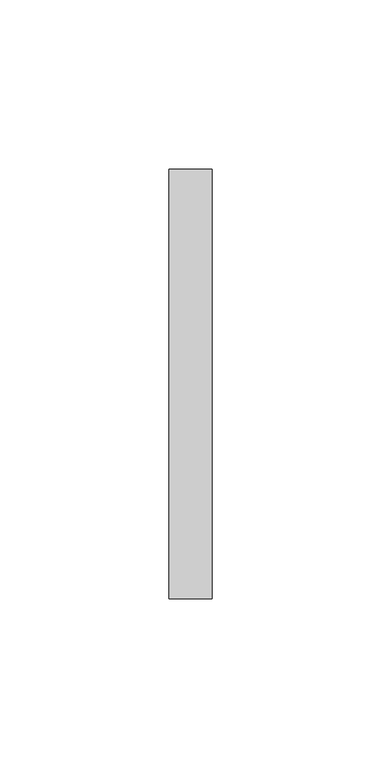
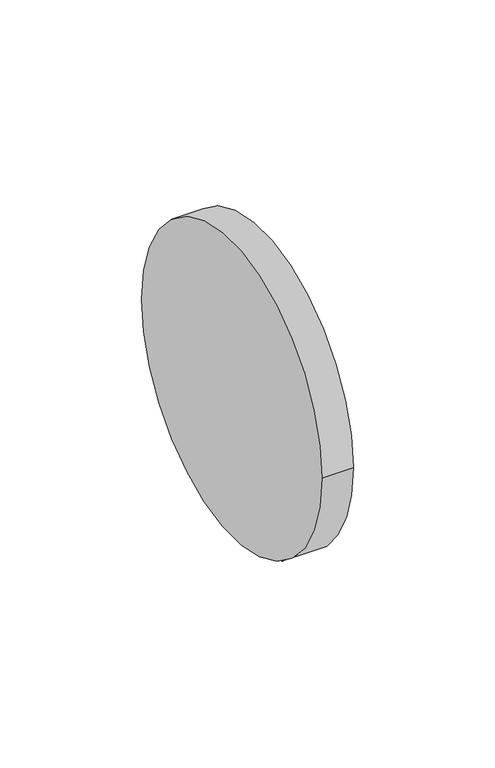
"""IFC4 building model written with IfcOpenShell, lengths in millimetres: proxy geometry, DOAS Supply to Return Connection : DOAS Supply to Return Duct Connection."""

import ifcopenshell
import ifcopenshell.guid

model = None  # the IFC model being written
_history = None  # IfcOwnerHistory: only IFC2X3 demands one
_inside = {}  # id of a spatial element -> (the spatial element, [elements in it])
_under = {}  # id of a project, library or spatial element -> (it, [spatial elements below it])
_declared = {}  # id of a project -> (the project, [libraries it declares])
_typed = {}  # id of a type object -> (the type object, [elements of that type])
_made_of = {}  # id of a material, layer set ... -> (it, [elements and type objects made of it])


def new_model(schema):
    """Start an empty IFC model of exactly this schema.

    Asked for "IFC4X3", IfcOpenShell would pick the latest addendum, in which some entities
    have other attributes; the version numbers below select the first issue.
    IFC2X3 requires an IfcOwnerHistory on every rooted entity: one is made here for all.
    """
    global model, _history
    if schema == "IFC4X3":
        model = ifcopenshell.file(schema_version=(4, 3, 0, 0))
    else:
        model = ifcopenshell.file(schema=schema)
    _inside.clear()
    _under.clear()
    _declared.clear()
    _typed.clear()
    _made_of.clear()
    _history = None
    if model.schema == "IFC2X3":
        org = make("IfcOrganization", Name="unknown")
        user = make(
            "IfcPersonAndOrganization",
            ThePerson=make("IfcPerson", FamilyName="unknown"),
            TheOrganization=org,
        )
        app = make(
            "IfcApplication",
            ApplicationDeveloper=org,
            Version="unknown",
            ApplicationFullName="unknown",
            ApplicationIdentifier="unknown",
        )
        _history = make(
            "IfcOwnerHistory",
            OwningUser=user,
            OwningApplication=app,
            ChangeAction="ADDED",
            CreationDate=0,
        )
    return model


def make(cls, **values):
    """One entity of the class cls with the attributes given. An attribute that is None is left unset."""
    return model.create_entity(
        cls, **{name: value for name, value in values.items() if value is not None}
    )


def rooted(cls, **values):
    """An entity with a GlobalId (a new one), such as an element, a storey or a relation."""
    return make(cls, GlobalId=ifcopenshell.guid.new(), OwnerHistory=_history, **values)


def si_unit(unit_type, name, prefix=None):
    """IfcSIUnit, for example si_unit("LENGTHUNIT", "METRE", prefix="MILLI")."""
    return make("IfcSIUnit", UnitType=unit_type, Prefix=prefix, Name=name)


def assignment(units):
    """IfcUnitAssignment: the units of a project."""
    return None if units is None else make("IfcUnitAssignment", Units=units)


def point(xyz):
    """IfcCartesianPoint."""
    return None if xyz is None else make("IfcCartesianPoint", Coordinates=xyz)


def direction(xyz):
    """IfcDirection."""
    return None if xyz is None else make("IfcDirection", DirectionRatios=xyz)


def frame(location, z_axis=None, x_axis=None):
    """IfcAxis2Placement3D, a coordinate frame: its origin and axes. An axis left out is left unset."""
    return make(
        "IfcAxis2Placement3D",
        Location=point(location),
        Axis=direction(z_axis),
        RefDirection=direction(x_axis),
    )


def frame_2d(location, x_axis=None):
    """IfcAxis2Placement2D, a coordinate frame in the plane: its origin and x axis."""
    return make(
        "IfcAxis2Placement2D", Location=point(location), RefDirection=direction(x_axis)
    )


def origin():
    """The frame at (0, 0, 0) with its axes left unset."""
    return frame((0.0, 0.0, 0.0))


def origin_2d():
    """The frame at (0, 0) in the plane with its x axis left unset."""
    return frame_2d((0.0, 0.0))


def place(relative_to, where):
    """IfcLocalPlacement: puts the frame where relative to a parent placement (None: the world)."""
    return make(
        "IfcLocalPlacement", PlacementRelTo=relative_to, RelativePlacement=where
    )


def context(
    kind, dimensions, precision=None, world=None, true_north=None, identifier=None
):
    """IfcGeometricRepresentationContext, for example the 3D "Model" context."""
    return make(
        "IfcGeometricRepresentationContext",
        ContextIdentifier=identifier,
        ContextType=kind,
        CoordinateSpaceDimension=dimensions,
        Precision=precision,
        WorldCoordinateSystem=world,
        TrueNorth=true_north,
    )


def project(units=None, contexts=None):
    """IfcProject with its units and contexts."""
    return rooted(
        "IfcProject",
        Name="project",
        RepresentationContexts=contexts,
        UnitsInContext=assignment(units),
    )


def spatial(cls, under=None, at=None, **own):
    """A site, building, storey or space (cls), placed at a placement, below another one or the project."""
    s = rooted(cls, ObjectPlacement=at, **own)
    if under is not None:
        _under.setdefault(under.id(), (under, []))[1].append(s)
    return s


def circle_curve(where, radius):
    """IfcCircle in the frame where."""
    return make("IfcCircle", Position=where, Radius=radius)


def trimmed(basis, trim1, trim2, sense, master):
    """IfcTrimmedCurve: the piece of a basis curve between two trims."""
    return make(
        "IfcTrimmedCurve",
        BasisCurve=basis,
        Trim1=trim1,
        Trim2=trim2,
        SenseAgreement=sense,
        MasterRepresentation=master,
    )


def segment(curve, same_sense, transition):
    """IfcCompositeCurveSegment."""
    return make(
        "IfcCompositeCurveSegment",
        Transition=transition,
        SameSense=same_sense,
        ParentCurve=curve,
    )


def composite_curve(segments, self_intersect=None):
    """IfcCompositeCurve: segments joined end to end."""
    return make("IfcCompositeCurve", Segments=segments, SelfIntersect=self_intersect)


def outline(outer, holes=None, kind="AREA"):
    """IfcArbitraryClosedProfileDef: a profile drawn as a closed curve; with holes, ...WithVoids."""
    if holes is None:
        return make("IfcArbitraryClosedProfileDef", ProfileType=kind, OuterCurve=outer)
    return make(
        "IfcArbitraryProfileDefWithVoids",
        ProfileType=kind,
        OuterCurve=outer,
        InnerCurves=holes,
    )


def extrude(swept, where, along, depth):
    """IfcExtrudedAreaSolid: the profile swept, set in the frame where, extruded along a direction by depth."""
    return make(
        "IfcExtrudedAreaSolid",
        SweptArea=swept,
        Position=where,
        ExtrudedDirection=direction(along),
        Depth=depth,
    )


def shape(context_of_items, identifier, shape_type, items):
    """IfcShapeRepresentation: the items that make up one representation, for example the "Body"."""
    return make(
        "IfcShapeRepresentation",
        ContextOfItems=context_of_items,
        RepresentationIdentifier=identifier,
        RepresentationType=shape_type,
        Items=items,
    )


def source(mapping_origin, context_of_items, identifier, shape_type, items):
    """IfcRepresentationMap: a shape defined once, which mapped items show again and again."""
    return make(
        "IfcRepresentationMap",
        MappingOrigin=mapping_origin,
        MappedRepresentation=shape(context_of_items, identifier, shape_type, items),
    )


def transform(
    local_origin,
    x_axis=None,
    y_axis=None,
    z_axis=None,
    scale=None,
    scale2=None,
    scale3=None,
    uniform=True,
):
    """IfcCartesianTransformationOperator3D, or its non-uniform kind. x_axis, y_axis, z_axis: its Axis1, 2, 3."""
    if uniform:
        return make(
            "IfcCartesianTransformationOperator3D",
            Axis1=direction(x_axis),
            Axis2=direction(y_axis),
            LocalOrigin=point(local_origin),
            Scale=scale,
            Axis3=direction(z_axis),
        )
    return make(
        "IfcCartesianTransformationOperator3DnonUniform",
        Axis1=direction(x_axis),
        Axis2=direction(y_axis),
        LocalOrigin=point(local_origin),
        Scale=scale,
        Axis3=direction(z_axis),
        Scale2=scale2,
        Scale3=scale3,
    )


def mapped(mapping_source, mapping_target):
    """IfcMappedItem: shows the shape of a source again, moved by a transform."""
    return make(
        "IfcMappedItem", MappingSource=mapping_source, MappingTarget=mapping_target
    )


def made_of(thing, what):
    """Note that an element or type object is made of a material, layer set ...; save() writes the relation."""
    if what is not None:
        _made_of.setdefault(what.id(), (what, []))[1].append(thing)
    return thing


def element(
    cls,
    number,
    at=None,
    inside=None,
    cuts=None,
    type_object=None,
    material=None,
    context=None,
    identifier="Body",
    shape_type=None,
    held_by="IfcProductDefinitionShape",
    body=None,
    shapes=None,
    **own,
):
    """One element of the class cls, such as IfcWall. Its Tag is "e" and its number.

    at: its placement. inside: the storey or other place that contains it. cuts: it is an
    opening in that element (IfcRelVoidsElement). A single representation is given by context,
    identifier, shape_type and body (its items); several are given by shapes. held_by: the class
    of the entity that holds the representations. save() writes the other relations.
    """
    e = rooted(cls, Tag="e%d" % number, ObjectPlacement=at, **own)
    if body is not None:
        shapes = [shape(context, identifier, shape_type, body)]
    if shapes is not None:
        e.Representation = make(held_by, Representations=shapes)
    if inside is not None:
        _inside.setdefault(inside.id(), (inside, []))[1].append(e)
    if cuts is not None:
        rooted(
            "IfcRelVoidsElement", RelatingBuildingElement=cuts, RelatedOpeningElement=e
        )
    if type_object is not None:
        _typed.setdefault(type_object.id(), (type_object, []))[1].append(e)
    return made_of(e, material)


def aggregate(whole, parts):
    """IfcRelAggregates: a whole, such as a stair, and the parts it consists of."""
    return rooted("IfcRelAggregates", RelatingObject=whole, RelatedObjects=parts)


def save(model, path):
    """Write the relations noted so far, then the file.

    IfcRelAggregates (storeys below a building ...), IfcRelContainedInSpatialStructure (elements
    in a storey), IfcRelDefinesByType, IfcRelAssociatesMaterial and IfcRelDeclares: one each for
    every whole, place, type object, material and project.
    """
    for whole, parts in _under.values():
        aggregate(whole, parts)
    for where, things in _inside.values():
        rooted(
            "IfcRelContainedInSpatialStructure",
            RelatedElements=things,
            RelatingStructure=where,
        )
    for kind, things in _typed.values():
        rooted("IfcRelDefinesByType", RelatedObjects=things, RelatingType=kind)
    for what, things in _made_of.values():
        rooted("IfcRelAssociatesMaterial", RelatedObjects=things, RelatingMaterial=what)
    for by, libraries in _declared.values():
        rooted("IfcRelDeclares", RelatingContext=by, RelatedDefinitions=libraries)
    model.write(path)


def mechanical_equipment_142123ad(model_context):
    return source(origin(), model_context, "Body", "SweptSolid", [
        extrude(outline(composite_curve([segment(trimmed(circle_curve(origin_2d(), 63.5), [point((-63.5, 0.0))], [point((63.5, 0.0))], False, "CARTESIAN"), True, "CONTINUOUS"), segment(trimmed(circle_curve(origin_2d(), 63.5), [point((63.5, 0.0))], [point((-63.5, 0.0))], False, "CARTESIAN"), True, "CONTINUOUS")], self_intersect=False)), frame((0.0, 0.0, 0.0), z_axis=(1.0, 0.0, 0.0), x_axis=(0.0, 1.0, 0.0)), (0.0, 0.0, 1.0), 12.7),
    ])


if __name__ == "__main__":
    model = new_model("IFC4")
    model_context = context("Model", 3, world=origin())
    ifc_project = project(units=[si_unit("LENGTHUNIT", "METRE", prefix="MILLI")], contexts=[model_context])
    site = spatial("IfcSite", under=ifc_project)
    building = spatial("IfcBuilding", under=site)
    placement = place(None, origin())
    mechanical_equipment_shape = mechanical_equipment_142123ad(model_context)
    element("IfcBuildingElementProxy", 1, Name="DOAS Supply to Return Connection : DOAS Supply to Return Duct Connection", ObjectType="DOAS Supply to Return Connection : DOAS Supply to Return Duct Connection", at=placement, inside=building, context=model_context, shape_type="MappedRepresentation", body=[
        mapped(mechanical_equipment_shape, transform((0.0, 0.0, 0.0), x_axis=(1.0, 0.0, 0.0), y_axis=(0.0, 1.0, 0.0), z_axis=(0.0, 0.0, 1.0))),
    ])
    save(model, "model.ifc")

# Revit data of these elements
# Type "DOAS Supply to Return Connection : DOAS Supply to Return Duct Connection"
#   Type Comments = "Generic Connector - no power"
#   Supply Side Airflow = 0 CFM
#   Return Side Airflow [instance default] = 0 CFM
#   Duct Connection [instance default] = 6"
#   Connector Length [instance default] = 12.7 mm
#   Default Elevation = 0
# Element 1 (IfcBuildingElementProxy, "DOAS Supply to Return Connection : DOAS Supply to Return Duct Connection")
#   Duct Connection = 5"
